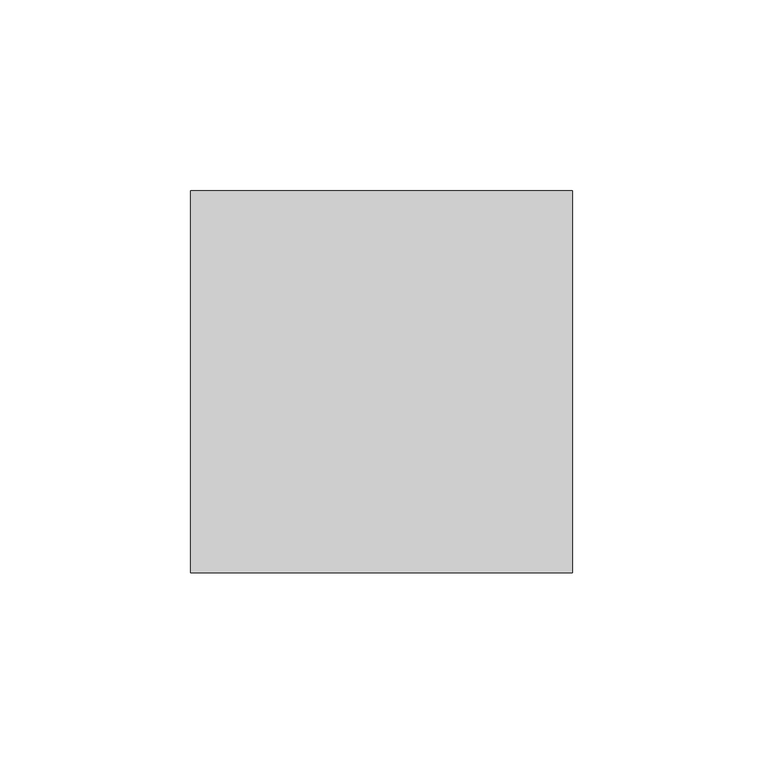
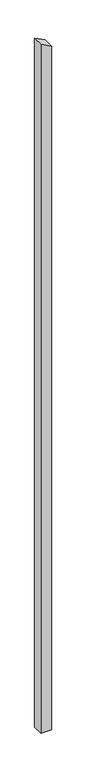
"""IFC4 building model written with IfcOpenShell, lengths in millimetres: column geometry, Holzstütze 159356 : Holzstütze 159356."""

import ifcopenshell
import ifcopenshell.guid

model = None  # the IFC model being written
_history = None  # IfcOwnerHistory: only IFC2X3 demands one
_inside = {}  # id of a spatial element -> (the spatial element, [elements in it])
_under = {}  # id of a project, library or spatial element -> (it, [spatial elements below it])
_declared = {}  # id of a project -> (the project, [libraries it declares])
_typed = {}  # id of a type object -> (the type object, [elements of that type])
_made_of = {}  # id of a material, layer set ... -> (it, [elements and type objects made of it])


def new_model(schema):
    """Start an empty IFC model of exactly this schema.

    Asked for "IFC4X3", IfcOpenShell would pick the latest addendum, in which some entities
    have other attributes; the version numbers below select the first issue.
    IFC2X3 requires an IfcOwnerHistory on every rooted entity: one is made here for all.
    """
    global model, _history
    if schema == "IFC4X3":
        model = ifcopenshell.file(schema_version=(4, 3, 0, 0))
    else:
        model = ifcopenshell.file(schema=schema)
    _inside.clear()
    _under.clear()
    _declared.clear()
    _typed.clear()
    _made_of.clear()
    _history = None
    if model.schema == "IFC2X3":
        org = make("IfcOrganization", Name="unknown")
        user = make(
            "IfcPersonAndOrganization",
            ThePerson=make("IfcPerson", FamilyName="unknown"),
            TheOrganization=org,
        )
        app = make(
            "IfcApplication",
            ApplicationDeveloper=org,
            Version="unknown",
            ApplicationFullName="unknown",
            ApplicationIdentifier="unknown",
        )
        _history = make(
            "IfcOwnerHistory",
            OwningUser=user,
            OwningApplication=app,
            ChangeAction="ADDED",
            CreationDate=0,
        )
    return model


def make(cls, **values):
    """One entity of the class cls with the attributes given. An attribute that is None is left unset."""
    return model.create_entity(
        cls, **{name: value for name, value in values.items() if value is not None}
    )


def rooted(cls, **values):
    """An entity with a GlobalId (a new one), such as an element, a storey or a relation."""
    return make(cls, GlobalId=ifcopenshell.guid.new(), OwnerHistory=_history, **values)


def si_unit(unit_type, name, prefix=None):
    """IfcSIUnit, for example si_unit("LENGTHUNIT", "METRE", prefix="MILLI")."""
    return make("IfcSIUnit", UnitType=unit_type, Prefix=prefix, Name=name)


def assignment(units):
    """IfcUnitAssignment: the units of a project."""
    return None if units is None else make("IfcUnitAssignment", Units=units)


def point(xyz):
    """IfcCartesianPoint."""
    return None if xyz is None else make("IfcCartesianPoint", Coordinates=xyz)


def direction(xyz):
    """IfcDirection."""
    return None if xyz is None else make("IfcDirection", DirectionRatios=xyz)


def frame(location, z_axis=None, x_axis=None):
    """IfcAxis2Placement3D, a coordinate frame: its origin and axes. An axis left out is left unset."""
    return make(
        "IfcAxis2Placement3D",
        Location=point(location),
        Axis=direction(z_axis),
        RefDirection=direction(x_axis),
    )


def origin():
    """The frame at (0, 0, 0) with its axes left unset."""
    return frame((0.0, 0.0, 0.0))


def place(relative_to, where):
    """IfcLocalPlacement: puts the frame where relative to a parent placement (None: the world)."""
    return make(
        "IfcLocalPlacement", PlacementRelTo=relative_to, RelativePlacement=where
    )


def context(
    kind, dimensions, precision=None, world=None, true_north=None, identifier=None
):
    """IfcGeometricRepresentationContext, for example the 3D "Model" context."""
    return make(
        "IfcGeometricRepresentationContext",
        ContextIdentifier=identifier,
        ContextType=kind,
        CoordinateSpaceDimension=dimensions,
        Precision=precision,
        WorldCoordinateSystem=world,
        TrueNorth=true_north,
    )


def project(units=None, contexts=None):
    """IfcProject with its units and contexts."""
    return rooted(
        "IfcProject",
        Name="project",
        RepresentationContexts=contexts,
        UnitsInContext=assignment(units),
    )


def spatial(cls, under=None, at=None, **own):
    """A site, building, storey or space (cls), placed at a placement, below another one or the project."""
    s = rooted(cls, ObjectPlacement=at, **own)
    if under is not None:
        _under.setdefault(under.id(), (under, []))[1].append(s)
    return s


def polyline(points):
    """IfcPolyline through the points."""
    return make("IfcPolyline", Points=[point(p) for p in points])


def outline(outer, holes=None, kind="AREA"):
    """IfcArbitraryClosedProfileDef: a profile drawn as a closed curve; with holes, ...WithVoids."""
    if holes is None:
        return make("IfcArbitraryClosedProfileDef", ProfileType=kind, OuterCurve=outer)
    return make(
        "IfcArbitraryProfileDefWithVoids",
        ProfileType=kind,
        OuterCurve=outer,
        InnerCurves=holes,
    )


def extrude(swept, where, along, depth):
    """IfcExtrudedAreaSolid: the profile swept, set in the frame where, extruded along a direction by depth."""
    return make(
        "IfcExtrudedAreaSolid",
        SweptArea=swept,
        Position=where,
        ExtrudedDirection=direction(along),
        Depth=depth,
    )


def shape(context_of_items, identifier, shape_type, items):
    """IfcShapeRepresentation: the items that make up one representation, for example the "Body"."""
    return make(
        "IfcShapeRepresentation",
        ContextOfItems=context_of_items,
        RepresentationIdentifier=identifier,
        RepresentationType=shape_type,
        Items=items,
    )


def source(mapping_origin, context_of_items, identifier, shape_type, items):
    """IfcRepresentationMap: a shape defined once, which mapped items show again and again."""
    return make(
        "IfcRepresentationMap",
        MappingOrigin=mapping_origin,
        MappedRepresentation=shape(context_of_items, identifier, shape_type, items),
    )


def transform(
    local_origin,
    x_axis=None,
    y_axis=None,
    z_axis=None,
    scale=None,
    scale2=None,
    scale3=None,
    uniform=True,
):
    """IfcCartesianTransformationOperator3D, or its non-uniform kind. x_axis, y_axis, z_axis: its Axis1, 2, 3."""
    if uniform:
        return make(
            "IfcCartesianTransformationOperator3D",
            Axis1=direction(x_axis),
            Axis2=direction(y_axis),
            LocalOrigin=point(local_origin),
            Scale=scale,
            Axis3=direction(z_axis),
        )
    return make(
        "IfcCartesianTransformationOperator3DnonUniform",
        Axis1=direction(x_axis),
        Axis2=direction(y_axis),
        LocalOrigin=point(local_origin),
        Scale=scale,
        Axis3=direction(z_axis),
        Scale2=scale2,
        Scale3=scale3,
    )


def mapped(mapping_source, mapping_target):
    """IfcMappedItem: shows the shape of a source again, moved by a transform."""
    return make(
        "IfcMappedItem", MappingSource=mapping_source, MappingTarget=mapping_target
    )


def made_of(thing, what):
    """Note that an element or type object is made of a material, layer set ...; save() writes the relation."""
    if what is not None:
        _made_of.setdefault(what.id(), (what, []))[1].append(thing)
    return thing


def element(
    cls,
    number,
    at=None,
    inside=None,
    cuts=None,
    type_object=None,
    material=None,
    context=None,
    identifier="Body",
    shape_type=None,
    held_by="IfcProductDefinitionShape",
    body=None,
    shapes=None,
    **own,
):
    """One element of the class cls, such as IfcWall. Its Tag is "e" and its number.

    at: its placement. inside: the storey or other place that contains it. cuts: it is an
    opening in that element (IfcRelVoidsElement). A single representation is given by context,
    identifier, shape_type and body (its items); several are given by shapes. held_by: the class
    of the entity that holds the representations. save() writes the other relations.
    """
    e = rooted(cls, Tag="e%d" % number, ObjectPlacement=at, **own)
    if body is not None:
        shapes = [shape(context, identifier, shape_type, body)]
    if shapes is not None:
        e.Representation = make(held_by, Representations=shapes)
    if inside is not None:
        _inside.setdefault(inside.id(), (inside, []))[1].append(e)
    if cuts is not None:
        rooted(
            "IfcRelVoidsElement", RelatingBuildingElement=cuts, RelatedOpeningElement=e
        )
    if type_object is not None:
        _typed.setdefault(type_object.id(), (type_object, []))[1].append(e)
    return made_of(e, material)


def aggregate(whole, parts):
    """IfcRelAggregates: a whole, such as a stair, and the parts it consists of."""
    return rooted("IfcRelAggregates", RelatingObject=whole, RelatedObjects=parts)


def save(model, path):
    """Write the relations noted so far, then the file.

    IfcRelAggregates (storeys below a building ...), IfcRelContainedInSpatialStructure (elements
    in a storey), IfcRelDefinesByType, IfcRelAssociatesMaterial and IfcRelDeclares: one each for
    every whole, place, type object, material and project.
    """
    for whole, parts in _under.values():
        aggregate(whole, parts)
    for where, things in _inside.values():
        rooted(
            "IfcRelContainedInSpatialStructure",
            RelatedElements=things,
            RelatingStructure=where,
        )
    for kind, things in _typed.values():
        rooted("IfcRelDefinesByType", RelatedObjects=things, RelatingType=kind)
    for what, things in _made_of.values():
        rooted("IfcRelAssociatesMaterial", RelatedObjects=things, RelatingMaterial=what)
    for by, libraries in _declared.values():
        rooted("IfcRelDeclares", RelatingContext=by, RelatedDefinitions=libraries)
    model.write(path)


def column_b2a6b517(model_context):
    return source(origin(), model_context, "Body", "SweptSolid", [
        extrude(outline(polyline([(-500.0, 174197.7593015), (-500.0, 174297.7593015), (6345.7118258, 174297.7593015), (6396.6643707, 174197.7593015), (-500.0, 174197.7593015)])), frame((0.0, 41761.7297978, 0.0), z_axis=(0.0, 1.0, 0.0), x_axis=(0.0, 0.0, 1.0)), (0.0, 0.0, 1.0), 100.0),
    ])


if __name__ == "__main__":
    model = new_model("IFC4")
    model_context = context("Model", 3, world=origin())
    ifc_project = project(units=[si_unit("LENGTHUNIT", "METRE", prefix="MILLI")], contexts=[model_context])
    site = spatial("IfcSite", under=ifc_project)
    building = spatial("IfcBuilding", under=site)
    placement = place(None, origin())
    column_shape = column_b2a6b517(model_context)
    element("IfcColumn", 1, ObjectType="Holzstütze 159356 : Holzstütze 159356", at=placement, inside=building, context=model_context, shape_type="MappedRepresentation", body=[
        mapped(column_shape, transform((0.0, 0.0, 0.0), x_axis=(1.0, 0.0, 0.0), y_axis=(0.0, 1.0, 0.0), z_axis=(0.0, 0.0, 1.0))),
    ])
    save(model, "model.ifc")

# Revit data of these elements
# Type "Holzstütze 159356 : Holzstütze 159356"
#   Abrechnungsart = "m"
#   Allright_Bauteil_ID = "0152St 0000143362"
#   Bezeichnung = "Holzstütze"
#   Codetext = "ST-HOLZ\\"
#   Gewerk = "Zimmer- und Holzbauarbeiten"
#   Material = "Holz"
#   Objektname = "Stütze"
#   NameOverride = "Holzstütze"
#   Reference = "Holzstütze"
#   Status = "NEW"
#   ThermalTransmittance = 0.0000 BTU/(h·ft²·°F)
#   Roll = 0.00°
#   Slope = 0.00°
#   2D Interaktion = yes
#   IsExternal = yes
#   LoadBearing = yes
# Element 1 (IfcColumn, "Holzstütze 159356 : Holzstütze 159356")
#   Materials on its faces: "holzschalung"
# Materials
#   "holzschalung": class "Unassigned", colour RGB 128 128 128, transparency 0
